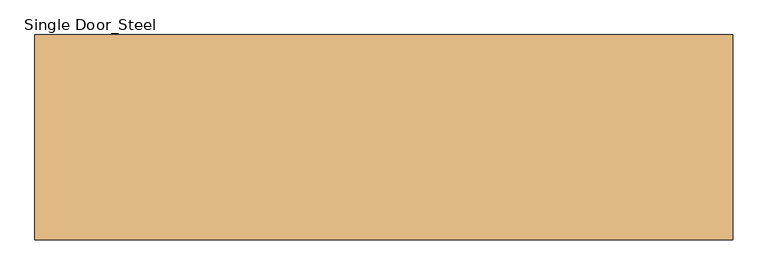
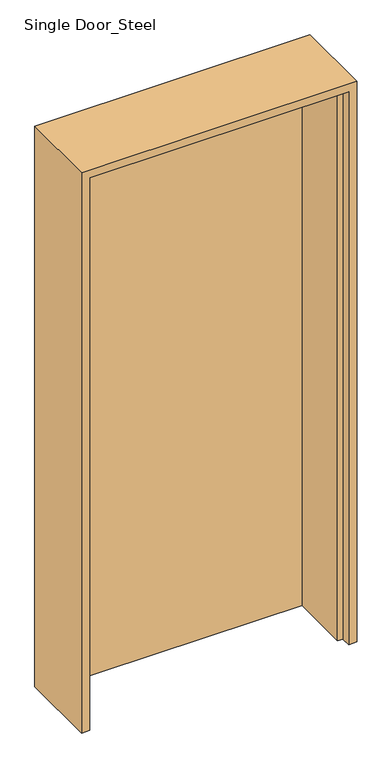
"""IFC4 building model written with IfcOpenShell, lengths in millimetres: door geometry, Single Door_Steel : H_DR_AMB_Single Door_Steel_W1000xH2150."""

from ifc_helpers import new_model, si_unit, origin, origin_with_axes, place, context, project, spatial, polyline, outline, extrude, faceted_brep, source, transform, mapped, element, save


def single_door_steel_d38beafa(model_context):
    return source(origin(), model_context, "Body", "SolidModel", [
        extrude(outline(polyline([(470.0, 147.0), (470.0, 112.0), (-470.0, 112.0), (-470.0, 147.0), (470.0, 147.0)])), origin_with_axes(), (0.0, 0.0, 1.0), 2120.0),
        faceted_brep([(470.0, 147.0, 0.0), (500.0, 147.0, 0.0), (500.0, -147.0, 0.0), (470.0, -147.0, 0.0), (470.0, -112.0, 0.0), (450.0, -112.0, 0.0), (450.0, 112.0, 0.0), (470.0, 112.0, 0.0), (470.0, 147.0, 2120.0), (-470.0, 147.0, 2120.0), (-470.0, 147.0, 0.0), (-500.0, 147.0, 0.0), (-500.0, 147.0, 2150.0), (500.0, 147.0, 2150.0), (500.0, -147.0, 2150.0), (-500.0, -147.0, 2150.0), (-500.0, -147.0, 0.0), (-470.0, -147.0, 0.0), (-470.0, -147.0, 2120.0), (470.0, -147.0, 2120.0), (470.0, -112.0, 2120.0), (-470.0, -112.0, 2120.0), (-470.0, -112.0, 0.0), (-450.0, -112.0, 0.0), (-450.0, -112.0, 2100.0), (450.0, -112.0, 2100.0), (450.0, 112.0, 2100.0), (-450.0, 112.0, 2100.0), (-450.0, 112.0, 0.0), (-470.0, 112.0, 0.0), (-470.0, 112.0, 2120.0), (470.0, 112.0, 2120.0)], [[[0, 1, 2, 3, 4, 5, 6, 7]], [[1, 0, 8, 9, 10, 11, 12, 13]], [[2, 1, 13, 14]], [[3, 2, 14, 15, 16, 17, 18, 19]], [[4, 3, 19, 20]], [[5, 4, 20, 21, 22, 23, 24, 25]], [[6, 5, 25, 26]], [[7, 6, 26, 27, 28, 29, 30, 31]], [[0, 7, 31, 8]], [[9, 30, 29, 10]], [[10, 29, 28, 23, 22, 17, 16, 11]], [[15, 12, 11, 16]], [[21, 18, 17, 22]], [[27, 24, 23, 28]], [[14, 13, 12, 15]], [[20, 19, 18, 21]], [[26, 25, 24, 27]], [[8, 31, 30, 9]]]),
    ])


if __name__ == "__main__":
    model = new_model("IFC4")
    model_context = context("Model", 3, world=origin())
    ifc_project = project(units=[si_unit("LENGTHUNIT", "METRE", prefix="MILLI")], contexts=[model_context])
    site = spatial("IfcSite", under=ifc_project)
    building = spatial("IfcBuilding", under=site)
    placement = place(None, origin())
    single_door_steel_shape = single_door_steel_d38beafa(model_context)
    element("IfcDoor", 1, ObjectType="Single Door_Steel : H_DR_AMB_Single Door_Steel_W1000xH2150", at=placement, inside=building, context=model_context, shape_type="MappedRepresentation", body=[
        mapped(single_door_steel_shape, transform((0.0, 0.0, 0.0), x_axis=(1.0, 0.0, 0.0), y_axis=(0.0, 1.0, 0.0), z_axis=(0.0, 0.0, 1.0))),
    ])
    save(model, "model.ifc")

# Revit data of these elements
# Type "Single Door_Steel : H_DR_AMB_Single Door_Steel_W1000xH2150"
#   Type Mark = "364"
#   Analytic Construction = "<None>"
#   프레임 투영 외부. = 25.000 mm
#   프레임 투영 내부. = 25.000 mm
#   프레임 폭 = 75.000 mm
#   Height = 2150.000 mm
#   Width = 1000.000 mm
#   Define Thermal Properties by = 1
#   문 패널 = none
#   문 프레임 = none
#   Function = (empty or 0)
#   Wall Closure = (empty or 0)
